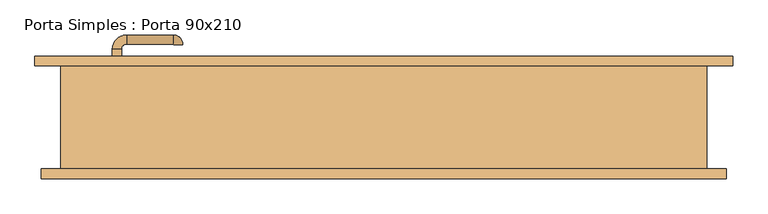
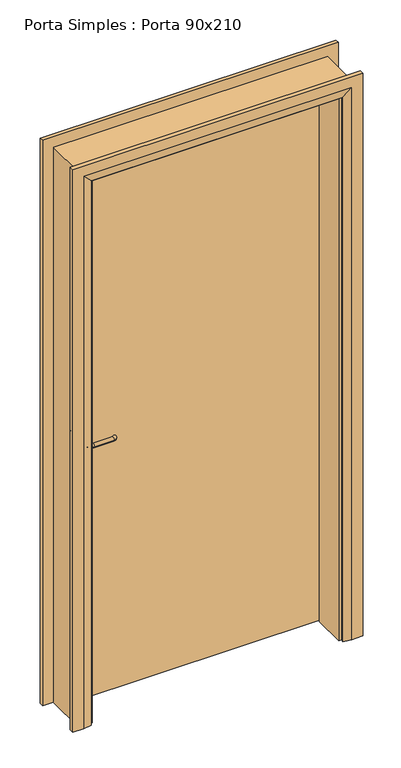
"""IFC4 building model written with IfcOpenShell, lengths in millimetres: door geometry, Porta Simples : Porta 90x210."""

from ifc_helpers import new_model, si_unit, point, frame, frame_2d, origin, place, context, project, spatial, polyline, circle_curve, ellipse_curve, trimmed, segment, composite_curve, outline, extrude, faceted_brep, source, transform, mapped, element, save
from ifc_brep_helpers import plane_surface, cylinder_surface, revolved_surface, advanced_brep


def porta_simples_porta_90x210_14889877(model_context):
    return source(origin(), model_context, "Body", "SolidModel", [
        extrude(outline(composite_curve([segment(trimmed(circle_curve(frame_2d((1050.0, -413.0)), 20.0), [point((1050.0, -433.0))], [point((1050.0, -393.0))], False, "CARTESIAN"), True, "CONTINUOUS"), segment(trimmed(circle_curve(frame_2d((1050.0, -413.0)), 20.0), [point((1050.0, -393.0))], [point((1050.0, -433.0))], False, "CARTESIAN"), True, "CONTINUOUS")], self_intersect=False)), frame((0.0, 34.0070105, 0.0), z_axis=(0.0, 1.0, 0.0), x_axis=(0.0, 0.0, 1.0)), (0.0, 0.0, 1.0), 4.5929895),
        advanced_brep(
        [(-406.0, 34.0070105, 1050.0), (-420.0, 34.0070105, 1050.0), (-420.0, 18.6, 1050.0), (-406.0, 18.6, 1050.0), (-398.0, -3.4, 1050.0), (-398.0, 10.6, 1050.0), (-326.0, -3.4, 1050.0), (-326.0, 10.6, 1050.0), (-325.0, 11.6, 1050.0), (-311.0, 11.6, 1050.0)],
        [
            (0, 1, circle_curve(frame((-413.0, 34.0070105, 1050.0), z_axis=(0.0, 1.0, 0.0), x_axis=(-1.0, 0.0, 0.0)), 7.0)),
            (1, 0, circle_curve(frame((-413.0, 34.0070105, 1050.0), z_axis=(0.0, 1.0, 0.0), x_axis=(-1.0, 0.0, 0.0)), 7.0)),
            (1, 2),
            (2, 3, circle_curve(frame((-413.0, 18.6, 1050.0), z_axis=(0.0, 1.0, 0.0), x_axis=(-1.0, 0.0, 0.0)), 7.0)),
            (3, 0),
            (3, 2, circle_curve(frame((-413.0, 18.6, 1050.0), z_axis=(0.0, 1.0, 0.0), x_axis=(-1.0, 0.0, 0.0)), 7.0)),
            (4, 5, circle_curve(frame((-398.0, 3.6, 1050.0), z_axis=(-1.0, 0.0, 0.0), x_axis=(0.0, -1.0, 0.0)), 7.0)),
            (5, 3, circle_curve(frame((-398.0, 18.6, 1050.0), z_axis=(0.0, 0.0, -1.0), x_axis=(-1.0, 0.0, 0.0)), 8.0)),
            (2, 4, circle_curve(frame((-398.0, 18.6, 1050.0), z_axis=(0.0, 0.0, 1.0), x_axis=(-1.0, 0.0, 0.0)), 22.0)),
            (5, 4, circle_curve(frame((-398.0, 3.6, 1050.0), z_axis=(-1.0, 0.0, 0.0), x_axis=(0.0, -1.0, 0.0)), 7.0)),
            (4, 6),
            (6, 7, circle_curve(frame((-326.0, 3.6, 1050.0), z_axis=(-1.0, 0.0, 0.0), x_axis=(0.0, -1.0, 0.0)), 7.0)),
            (7, 5),
            (7, 6, circle_curve(frame((-326.0, 3.6, 1050.0), z_axis=(-1.0, 0.0, 0.0), x_axis=(0.0, -1.0, 0.0)), 7.0)),
            (8, 9, circle_curve(frame((-318.0, 11.6, 1050.0), z_axis=(0.0, 1.0, 0.0), x_axis=(1.0, 0.0, 0.0)), 7.0)),
            (9, 8, circle_curve(frame((-318.0, 11.6, 1050.0), z_axis=(0.0, 1.0, 0.0), x_axis=(1.0, 0.0, 0.0)), 7.0)),
            (8, 7, circle_curve(frame((-326.0, 11.6, 1050.0), z_axis=(0.0, 0.0, -1.0), x_axis=(0.0, -1.0, 0.0)), 1.0)),
            (6, 9, circle_curve(frame((-326.0, 11.6, 1050.0), z_axis=(0.0, 0.0, 1.0), x_axis=(0.0, -1.0, 0.0)), 15.0)),
        ],
        [
            plane_surface(frame((-413.0, 34.0070105, 1050.0), z_axis=(0.0, 1.0, 0.0), x_axis=(0.0, 0.0, 1.0))),
            cylinder_surface(frame((-413.0, 34.0070105, 1050.0), z_axis=(0.0, 1.0, 0.0), x_axis=(-1.0, 0.0, 0.0)), 7.0),
            revolved_surface(trimmed(ellipse_curve(frame((-413.0, 18.6, 1050.0), z_axis=(0.0, -1.0, 0.0), x_axis=(-1.0, 0.0, 0.0)), 7.0, 7.0), [point((-406.0, 18.6, 1050.0))], [point((-420.0, 18.6, 1050.0))], True, "CARTESIAN"), (-398.0, 18.6, 1050.0), (0.0, 0.0, -1.0)),
            revolved_surface(trimmed(ellipse_curve(frame((-413.0, 18.6, 1050.0), z_axis=(0.0, -1.0, 0.0), x_axis=(-1.0, 0.0, 0.0)), 7.0, 7.0), [point((-420.0, 18.6, 1050.0))], [point((-406.0, 18.6, 1050.0))], True, "CARTESIAN"), (-398.0, 18.6, 1050.0), (0.0, 0.0, -1.0)),
            cylinder_surface(frame((-398.0, 3.6, 1050.0), z_axis=(-1.0, 0.0, 0.0), x_axis=(0.0, -1.0, 0.0)), 7.0),
            plane_surface(frame((-318.0, 11.6, 1050.0), z_axis=(0.0, 1.0, 0.0), x_axis=(0.0, 0.0, 1.0))),
            revolved_surface(trimmed(ellipse_curve(frame((-326.0, 3.6, 1050.0), z_axis=(1.0, 0.0, 0.0), x_axis=(0.0, -1.0, 0.0)), 7.0, 7.0), [point((-326.0, 10.6, 1050.0))], [point((-326.0, -3.4, 1050.0))], True, "CARTESIAN"), (-326.0, 11.6, 1050.0), (0.0, 0.0, -1.0)),
            revolved_surface(trimmed(ellipse_curve(frame((-326.0, 3.6, 1050.0), z_axis=(1.0, 0.0, 0.0), x_axis=(0.0, -1.0, 0.0)), 7.0, 7.0), [point((-326.0, -3.4, 1050.0))], [point((-326.0, 10.6, 1050.0))], True, "CARTESIAN"), (-326.0, 11.6, 1050.0), (0.0, 0.0, -1.0)),
        ],
        [
            (0, [[1, 2]]),
            (1, [[3, 4, 5, -2]]),
            (1, [[-5, 6, -3, -1]]),
            (2, [[7, 8, -4, 9]]),
            (3, [[10, -9, -6, -8]]),
            (4, [[11, 12, 13, -7]]),
            (4, [[-13, 14, -11, -10]]),
            (5, [[15, 16]]),
            (6, [[-15, 17, -12, 18]]),
            (7, [[-16, -18, -14, -17]]),
        ],
    ),
        extrude(outline(polyline([(-383.0, 44.6), (-383.0, 38.6), (-443.0, 38.6), (-443.0, 44.6), (-383.0, 44.6)])), frame((0.0, 0.0, 925.0), z_axis=(0.0, 0.0, 1.0), x_axis=(1.0, 0.0, 0.0)), (0.0, 0.0, 1.0), 165.0),
        extrude(outline(composite_curve([segment(trimmed(circle_curve(frame_2d((1050.0, -413.0)), 20.0), [point((1050.0, -433.0))], [point((1050.0, -393.0))], False, "CARTESIAN"), True, "CONTINUOUS"), segment(trimmed(circle_curve(frame_2d((1050.0, -413.0)), 20.0), [point((1050.0, -393.0))], [point((1050.0, -433.0))], False, "CARTESIAN"), True, "CONTINUOUS")], self_intersect=False)), frame((0.0, 85.6, 0.0), z_axis=(0.0, 1.0, 0.0), x_axis=(0.0, 0.0, 1.0)), (0.0, 0.0, 1.0), 4.5929895),
        advanced_brep(
        [(-406.0, 90.1929895, 1050.0), (-420.0, 90.1929895, 1050.0), (-406.0, 105.6, 1050.0), (-420.0, 105.6, 1050.0), (-398.0, 127.6, 1050.0), (-398.0, 113.6, 1050.0), (-326.0, 113.6, 1050.0), (-326.0, 127.6, 1050.0), (-325.0, 112.6, 1050.0), (-311.0, 112.6, 1050.0)],
        [
            (0, 1, circle_curve(frame((-413.0, 90.1929895, 1050.0), z_axis=(0.0, -1.0, 0.0), x_axis=(-1.0, 0.0, 0.0)), 7.0)),
            (1, 0, circle_curve(frame((-413.0, 90.1929895, 1050.0), z_axis=(0.0, -1.0, 0.0), x_axis=(-1.0, 0.0, 0.0)), 7.0)),
            (0, 2),
            (2, 3, circle_curve(frame((-413.0, 105.6, 1050.0), z_axis=(0.0, -1.0, 0.0), x_axis=(-1.0, 0.0, 0.0)), 7.0)),
            (3, 1),
            (3, 2, circle_curve(frame((-413.0, 105.6, 1050.0), z_axis=(0.0, -1.0, 0.0), x_axis=(-1.0, 0.0, 0.0)), 7.0)),
            (4, 3, circle_curve(frame((-398.0, 105.6, 1050.0), z_axis=(0.0, 0.0, 1.0), x_axis=(-1.0, 0.0, 0.0)), 22.0)),
            (2, 5, circle_curve(frame((-398.0, 105.6, 1050.0), z_axis=(0.0, 0.0, -1.0), x_axis=(-1.0, 0.0, 0.0)), 8.0)),
            (5, 4, circle_curve(frame((-398.0, 120.6, 1050.0), z_axis=(-1.0, 0.0, 0.0), x_axis=(0.0, 1.0, 0.0)), 7.0)),
            (4, 5, circle_curve(frame((-398.0, 120.6, 1050.0), z_axis=(-1.0, 0.0, 0.0), x_axis=(0.0, 1.0, 0.0)), 7.0)),
            (5, 6),
            (6, 7, circle_curve(frame((-326.0, 120.6, 1050.0), z_axis=(-1.0, 0.0, 0.0), x_axis=(0.0, 1.0, 0.0)), 7.0)),
            (7, 4),
            (7, 6, circle_curve(frame((-326.0, 120.6, 1050.0), z_axis=(-1.0, 0.0, 0.0), x_axis=(0.0, 1.0, 0.0)), 7.0)),
            (8, 9, circle_curve(frame((-318.0, 112.6, 1050.0), z_axis=(0.0, -1.0, 0.0), x_axis=(1.0, 0.0, 0.0)), 7.0)),
            (9, 8, circle_curve(frame((-318.0, 112.6, 1050.0), z_axis=(0.0, -1.0, 0.0), x_axis=(1.0, 0.0, 0.0)), 7.0)),
            (9, 7, circle_curve(frame((-326.0, 112.6, 1050.0), z_axis=(0.0, 0.0, 1.0), x_axis=(0.0, 1.0, 0.0)), 15.0)),
            (6, 8, circle_curve(frame((-326.0, 112.6, 1050.0), z_axis=(0.0, 0.0, -1.0), x_axis=(0.0, 1.0, 0.0)), 1.0)),
        ],
        [
            plane_surface(frame((-413.0, 90.1929895, 1050.0), z_axis=(0.0, -1.0, 0.0), x_axis=(0.0, 0.0, 1.0))),
            cylinder_surface(frame((-413.0, 90.1929895, 1050.0), z_axis=(0.0, -1.0, 0.0), x_axis=(-1.0, 0.0, 0.0)), 7.0),
            revolved_surface(trimmed(ellipse_curve(frame((-413.0, 105.6, 1050.0), z_axis=(0.0, -1.0, 0.0), x_axis=(-1.0, 0.0, 0.0)), 7.0, 7.0), [point((-406.0, 105.6, 1050.0))], [point((-420.0, 105.6, 1050.0))], True, "CARTESIAN"), (-398.0, 105.6, 1050.0), (0.0, 0.0, -1.0)),
            revolved_surface(trimmed(ellipse_curve(frame((-413.0, 105.6, 1050.0), z_axis=(0.0, -1.0, 0.0), x_axis=(-1.0, 0.0, 0.0)), 7.0, 7.0), [point((-420.0, 105.6, 1050.0))], [point((-406.0, 105.6, 1050.0))], True, "CARTESIAN"), (-398.0, 105.6, 1050.0), (0.0, 0.0, -1.0)),
            cylinder_surface(frame((-398.0, 120.6, 1050.0), z_axis=(-1.0, 0.0, 0.0), x_axis=(0.0, 1.0, 0.0)), 7.0),
            plane_surface(frame((-318.0, 112.6, 1050.0), z_axis=(0.0, -1.0, 0.0), x_axis=(0.0, 0.0, 1.0))),
            revolved_surface(trimmed(ellipse_curve(frame((-326.0, 120.6, 1050.0), z_axis=(-1.0, 0.0, 0.0), x_axis=(0.0, 1.0, 0.0)), 7.0, 7.0), [point((-326.0, 113.6, 1050.0))], [point((-326.0, 127.6, 1050.0))], True, "CARTESIAN"), (-326.0, 112.6, 1050.0), (0.0, 0.0, -1.0)),
            revolved_surface(trimmed(ellipse_curve(frame((-326.0, 120.6, 1050.0), z_axis=(-1.0, 0.0, 0.0), x_axis=(0.0, 1.0, 0.0)), 7.0, 7.0), [point((-326.0, 127.6, 1050.0))], [point((-326.0, 113.6, 1050.0))], True, "CARTESIAN"), (-326.0, 112.6, 1050.0), (0.0, 0.0, -1.0)),
        ],
        [
            (0, [[1, 2]]),
            (1, [[-1, 3, 4, 5]]),
            (1, [[-2, -5, 6, -3]]),
            (2, [[7, -4, 8, 9]]),
            (3, [[-8, -6, -7, 10]]),
            (4, [[-9, 11, 12, 13]]),
            (4, [[-10, -13, 14, -11]]),
            (5, [[15, 16]]),
            (6, [[17, -12, 18, -16]]),
            (7, [[-18, -14, -17, -15]]),
        ],
    ),
        extrude(outline(polyline([(-383.0, 79.6), (-443.0, 79.6), (-443.0, 85.6), (-383.0, 85.6), (-383.0, 79.6)])), frame((0.0, 0.0, 925.0), z_axis=(0.0, 0.0, 1.0), x_axis=(1.0, 0.0, 0.0)), (0.0, 0.0, 1.0), 165.0),
        extrude(outline(polyline([(457.0, 44.6), (-457.0, 44.6), (-457.0, 79.6), (457.0, 79.6), (457.0, 44.6)])), frame((0.0, 0.0, 53.0), z_axis=(0.0, 0.0, 1.0), x_axis=(1.0, 0.0, 0.0)), (0.0, 0.0, 1.0), 2094.0),
        faceted_brep([(530.0, -79.6, 50.0), (530.0, -94.6, 50.0), (490.0, -94.6, 50.0), (460.0, -89.6, 50.0), (460.0, -79.6, 50.0), (530.0, -79.6, 2220.0), (530.0, -94.6, 2220.0), (-530.0, -94.6, 2220.0), (-530.0, -94.6, 50.0), (-490.0, -94.6, 50.0), (-490.0, -94.6, 2180.0), (490.0, -94.6, 2180.0), (460.0, -89.6, 2150.0), (460.0, -79.6, 2150.0), (-460.0, -79.6, 2150.0), (-460.0, -79.6, 50.0), (-530.0, -79.6, 50.0), (-530.0, -79.6, 2220.0), (-460.0, -89.6, 2150.0), (-460.0, -89.6, 50.0)], [[[0, 1, 2, 3, 4]], [[1, 0, 5, 6]], [[2, 1, 6, 7, 8, 9, 10, 11]], [[3, 2, 11, 12]], [[4, 3, 12, 13]], [[0, 4, 13, 14, 15, 16, 17, 5]], [[14, 18, 19, 15]], [[16, 15, 19, 9, 8]], [[7, 17, 16, 8]], [[18, 10, 9, 19]], [[13, 12, 18, 14]], [[6, 5, 17, 7]], [[12, 11, 10, 18]]]),
        faceted_brep([(540.0, 79.6, 50.0), (470.0, 79.6, 50.0), (470.0, 89.6, 50.0), (500.0, 94.6, 50.0), (540.0, 94.6, 50.0), (540.0, 79.6, 2230.0), (-540.0, 79.6, 2230.0), (-540.0, 79.6, 50.0), (-470.0, 79.6, 50.0), (-470.0, 79.6, 2160.0), (470.0, 79.6, 2160.0), (470.0, 89.6, 2160.0), (500.0, 94.6, 2190.0), (-500.0, 94.6, 2190.0), (-500.0, 94.6, 50.0), (-540.0, 94.6, 50.0), (-540.0, 94.6, 2230.0), (540.0, 94.6, 2230.0), (-470.0, 89.6, 50.0), (-470.0, 89.6, 2160.0)], [[[0, 1, 2, 3, 4]], [[1, 0, 5, 6, 7, 8, 9, 10]], [[2, 1, 10, 11]], [[3, 2, 11, 12]], [[4, 3, 12, 13, 14, 15, 16, 17]], [[0, 4, 17, 5]], [[6, 16, 15, 7]], [[7, 15, 14, 18, 8]], [[19, 9, 8, 18]], [[13, 19, 18, 14]], [[11, 10, 9, 19]], [[5, 17, 16, 6]], [[12, 11, 19, 13]]]),
        faceted_brep([(-460.0, 79.6, 50.0), (-460.0, 41.6, 50.0), (-450.0, 41.6, 50.0), (-450.0, -79.6, 50.0), (-500.0, -79.6, 50.0), (-500.0, 79.6, 50.0), (-460.0, 79.6, 2150.0), (-460.0, 41.6, 2150.0), (-450.0, 41.6, 2140.0), (-450.0, -79.6, 2140.0), (-500.0, -79.6, 2190.0), (-500.0, 79.6, 2190.0), (460.0, 79.6, 50.0), (500.0, 79.6, 50.0), (500.0, -79.6, 50.0), (450.0, -79.6, 50.0), (450.0, 41.6, 50.0), (460.0, 41.6, 50.0), (460.0, 79.6, 2150.0), (500.0, 79.6, 2190.0), (500.0, -79.6, 2190.0), (450.0, -79.6, 2140.0), (450.0, 41.6, 2140.0), (460.0, 41.6, 2150.0)], [[[0, 1, 2, 3, 4, 5]], [[1, 0, 6, 7]], [[2, 1, 7, 8]], [[3, 2, 8, 9]], [[4, 3, 9, 10]], [[5, 4, 10, 11]], [[0, 5, 11, 6]], [[12, 13, 14, 15, 16, 17]], [[18, 19, 13, 12]], [[19, 20, 14, 13]], [[20, 21, 15, 14]], [[21, 22, 16, 15]], [[22, 23, 17, 16]], [[23, 18, 12, 17]], [[7, 6, 18, 23]], [[8, 7, 23, 22]], [[9, 8, 22, 21]], [[10, 9, 21, 20]], [[11, 10, 20, 19]], [[6, 11, 19, 18]]]),
    ])


if __name__ == "__main__":
    model = new_model("IFC4")
    model_context = context("Model", 3, world=origin())
    ifc_project = project(units=[si_unit("LENGTHUNIT", "METRE", prefix="MILLI")], contexts=[model_context])
    site = spatial("IfcSite", under=ifc_project)
    building = spatial("IfcBuilding", under=site)
    placement = place(None, origin())
    porta_simples_porta_90x210_shape = porta_simples_porta_90x210_14889877(model_context)
    element("IfcDoor", 1, ObjectType="Porta Simples : Porta 90x210", at=placement, inside=building, context=model_context, shape_type="MappedRepresentation", body=[
        mapped(porta_simples_porta_90x210_shape, transform((0.0, 0.0, 0.0), x_axis=(1.0, 0.0, 0.0), y_axis=(0.0, 1.0, 0.0), z_axis=(0.0, 0.0, 1.0))),
    ])
    save(model, "model.ifc")

# Revit data of these elements
# Type "Porta Simples : Porta 90x210"
#   Type Mark = "48"
#   SINAPI = ""
#   Analytic Construction = "<Nenhum>"
#   Construction Type = "300"
#   Maçaneta [instance default] = ""
#   Fechadura [instance default] = ""
#   Vão Luz (somente para informação) = 0.88 m
#   Tolerância Folha Vertical = 0.003 m
#   Módulo Básico M = 0.10 m
#   Largura de Coordenação Modular Largura CM = 1.00 m
#   Rough Width = 1.00 m
#   Deslocamento da Horizontal da Folha = 0.00 m
#   Altura de Coordenação Modular Largura CM = 2.20 m
#   Rough Height = 2.20 m
#   Altura Nominal = 2.09 m
#   Ajuste de Coordenação Topo AC Topo = 0.01 m
#   Ajuste de Coordenação Base AC Base = 0.05 m
#   Ajuste de Coordenação AC = 0.01 m
#   Tolerância Folha Horizontal = 0.003 m
#   Largura Folha (somente para informação) = 0.894 m
#   Espessura Folha = 0.035 m
#   Maçaneta - Distância da Folha = 0.044 m
#   Maçaneta - Altura = 1.00 m
#   Largura Nominal (Largura Mn) = 0.92 m
#   Distância do Nível = 0.003 m
#   Aduela Interna Espessura = 0.04 m
#   Aduela Externa Espessura = 0.05 m
#   Altura Folha (somente para informação) = 2.074 m
#   Height = 2.14 m
#   Width = 0.98 m
#   Número de Módulos Básicos nM Largura = 10
#   Número de Módulos Básicos nM Altura = 22
#   Marco Metálico = no
#   Aduela de Madeira = no
#   Aduela Metálica de Canto = no
#   Guarnição Reta = no
#   Guarnição Chanfrada = yes
#   Batente - Material [instance default] = none
#   Painel - Material [instance default] = none
#   Model = ""
#   Function = (empty or 0)
#   Description = (empty or 0)
#   Wall Closure = (empty or 0)
#   Assembly Code = ""
# Element 1 (IfcDoor, "Porta Simples : Porta 90x210")
#   Materials on its faces: "Porta - Maçaneta"
# Materials
#   "Porta - Maçaneta": class "Diversos", colour RGB 0 0 0, transparency 0
